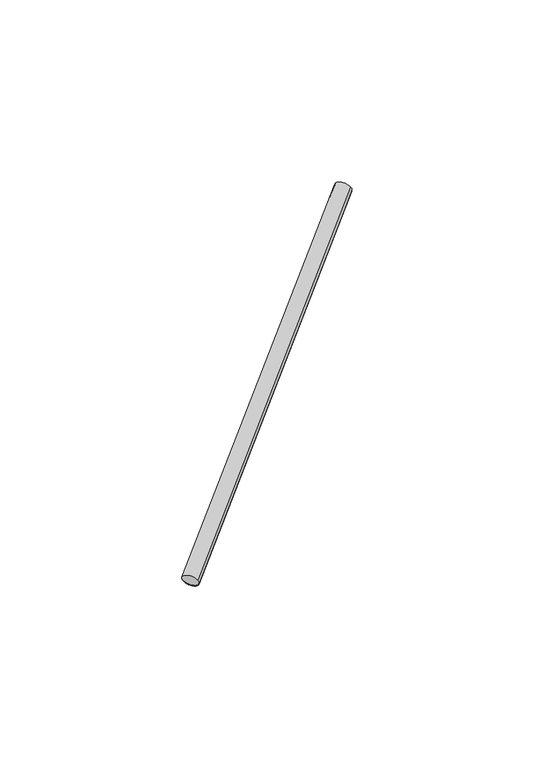
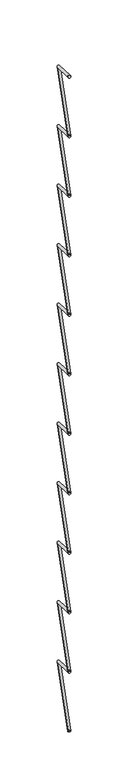
"""IFC4 building model written with IfcOpenShell, lengths in millimetres: proxy geometry, Vigota 2 (Pano 4) (Mf = 837)."""

from ifc_helpers import new_model, si_unit, point, frame, origin, origin_2d, place, context, project, spatial, circle_curve, trimmed, segment, composite_curve, outline, extrude, source, transform, mapped, element, save


def structural_framing_aa4d0655(model_context):
    return source(origin(), model_context, "Body", "SweptSolid", [
        extrude(outline(composite_curve([segment(trimmed(circle_curve(origin_2d(), 2.5), [point((2.5, 0.0))], [point((-2.5, 0.0))], False, "CARTESIAN"), True, "CONTINUOUS"), segment(trimmed(circle_curve(origin_2d(), 2.5), [point((-2.5, 0.0))], [point((2.5, 0.0))], False, "CARTESIAN"), True, "CONTINUOUS")], self_intersect=False)), frame((-42.0, 0.0, 1765.0), z_axis=(0.3218603428886276, 0.8276408817707567, 0.4598004898837537), x_axis=(0.8192319205108605, 3.936835275445103e-11, -0.5734623443750141)), (0.0, 0.0, 1.0), 130.491379),
        extrude(outline(composite_curve([segment(trimmed(circle_curve(origin_2d(), 2.5), [point((2.5, 0.0))], [point((-2.5, 0.0))], False, "CARTESIAN"), True, "CONTINUOUS"), segment(trimmed(circle_curve(origin_2d(), 2.5), [point((-2.5, 0.0))], [point((2.5, 0.0))], False, "CARTESIAN"), True, "CONTINUOUS")], self_intersect=False)), frame((0.0, 108.0, 1825.0), z_axis=(-0.3218603428886276, -0.8276408817707567, 0.4598004898837537), x_axis=(0.8192319205108605, 3.936835275445103e-11, 0.5734623443750141)), (0.0, 0.0, 1.0), 130.491379),
        extrude(outline(composite_curve([segment(trimmed(circle_curve(origin_2d(), 2.5), [point((2.5, 0.0))], [point((-2.5, 0.0))], False, "CARTESIAN"), True, "CONTINUOUS"), segment(trimmed(circle_curve(origin_2d(), 2.5), [point((-2.5, 0.0))], [point((2.5, 0.0))], False, "CARTESIAN"), True, "CONTINUOUS")], self_intersect=False)), frame((-42.0, 0.0, 1885.0), z_axis=(0.3218603428886276, 0.8276408817707567, 0.4598004898837537), x_axis=(0.8192319205108605, 3.936835275445103e-11, -0.5734623443750141)), (0.0, 0.0, 1.0), 130.491379),
        extrude(outline(composite_curve([segment(trimmed(circle_curve(origin_2d(), 2.5), [point((2.5, 0.0))], [point((-2.5, 0.0))], False, "CARTESIAN"), True, "CONTINUOUS"), segment(trimmed(circle_curve(origin_2d(), 2.5), [point((-2.5, 0.0))], [point((2.5, 0.0))], False, "CARTESIAN"), True, "CONTINUOUS")], self_intersect=False)), frame((0.0, 108.0, 1945.0), z_axis=(-0.3218603428886276, -0.8276408817707567, 0.4598004898837537), x_axis=(0.8192319205108605, 3.936835275445103e-11, 0.5734623443750141)), (0.0, 0.0, 1.0), 130.491379),
        extrude(outline(composite_curve([segment(trimmed(circle_curve(origin_2d(), 2.5), [point((2.5, 0.0))], [point((-2.5, 0.0))], False, "CARTESIAN"), True, "CONTINUOUS"), segment(trimmed(circle_curve(origin_2d(), 2.5), [point((-2.5, 0.0))], [point((2.5, 0.0))], False, "CARTESIAN"), True, "CONTINUOUS")], self_intersect=False)), frame((-42.0, 0.0, 2005.0), z_axis=(0.3218603428886276, 0.8276408817707567, 0.4598004898837537), x_axis=(0.8192319205108605, 3.936835275445103e-11, -0.5734623443750141)), (0.0, 0.0, 1.0), 130.491379),
        extrude(outline(composite_curve([segment(trimmed(circle_curve(origin_2d(), 2.5), [point((2.5, 0.0))], [point((-2.5, 0.0))], False, "CARTESIAN"), True, "CONTINUOUS"), segment(trimmed(circle_curve(origin_2d(), 2.5), [point((-2.5, 0.0))], [point((2.5, 0.0))], False, "CARTESIAN"), True, "CONTINUOUS")], self_intersect=False)), frame((0.0, 108.0, 2065.0), z_axis=(-0.3218603428886276, -0.8276408817707567, 0.4598004898837537), x_axis=(0.8192319205108605, 3.936835275445103e-11, 0.5734623443750141)), (0.0, 0.0, 1.0), 130.491379),
        extrude(outline(composite_curve([segment(trimmed(circle_curve(origin_2d(), 2.5), [point((2.5, 0.0))], [point((-2.5, 0.0))], False, "CARTESIAN"), True, "CONTINUOUS"), segment(trimmed(circle_curve(origin_2d(), 2.5), [point((-2.5, 0.0))], [point((2.5, 0.0))], False, "CARTESIAN"), True, "CONTINUOUS")], self_intersect=False)), frame((-42.0, 0.0, 2125.0), z_axis=(0.3218603428886276, 0.8276408817707567, 0.4598004898837537), x_axis=(0.8192319205108605, 3.936835275445103e-11, -0.5734623443750141)), (0.0, 0.0, 1.0), 130.491379),
        extrude(outline(composite_curve([segment(trimmed(circle_curve(origin_2d(), 2.5), [point((2.5, 0.0))], [point((-2.5, 0.0))], False, "CARTESIAN"), True, "CONTINUOUS"), segment(trimmed(circle_curve(origin_2d(), 2.5), [point((-2.5, 0.0))], [point((2.5, 0.0))], False, "CARTESIAN"), True, "CONTINUOUS")], self_intersect=False)), frame((0.0, 108.0, 2185.0), z_axis=(-0.3218603428886276, -0.8276408817707567, 0.4598004898837537), x_axis=(0.8192319205108605, 3.936835275445103e-11, 0.5734623443750141)), (0.0, 0.0, 1.0), 130.491379),
        extrude(outline(composite_curve([segment(trimmed(circle_curve(origin_2d(), 2.5), [point((2.5, 0.0))], [point((-2.5, 0.0))], False, "CARTESIAN"), True, "CONTINUOUS"), segment(trimmed(circle_curve(origin_2d(), 2.5), [point((-2.5, 0.0))], [point((2.5, 0.0))], False, "CARTESIAN"), True, "CONTINUOUS")], self_intersect=False)), frame((-42.0, 0.0, 2245.0), z_axis=(0.3218603428886276, 0.8276408817707567, 0.4598004898837537), x_axis=(0.8192319205108605, 3.936835275445103e-11, -0.5734623443750141)), (0.0, 0.0, 1.0), 130.491379),
        extrude(outline(composite_curve([segment(trimmed(circle_curve(origin_2d(), 2.5), [point((2.5, 0.0))], [point((-2.5, 0.0))], False, "CARTESIAN"), True, "CONTINUOUS"), segment(trimmed(circle_curve(origin_2d(), 2.5), [point((-2.5, 0.0))], [point((2.5, 0.0))], False, "CARTESIAN"), True, "CONTINUOUS")], self_intersect=False)), frame((0.0, 108.0, 2305.0), z_axis=(-0.3218603428886276, -0.8276408817707567, 0.4598004898837537), x_axis=(0.8192319205108605, 3.936835275445103e-11, 0.5734623443750141)), (0.0, 0.0, 1.0), 130.491379),
        extrude(outline(composite_curve([segment(trimmed(circle_curve(origin_2d(), 2.5), [point((2.5, 0.0))], [point((-2.5, 0.0))], False, "CARTESIAN"), True, "CONTINUOUS"), segment(trimmed(circle_curve(origin_2d(), 2.5), [point((-2.5, 0.0))], [point((2.5, 0.0))], False, "CARTESIAN"), True, "CONTINUOUS")], self_intersect=False)), frame((-42.0, 0.0, 2365.0), z_axis=(0.3218603428886276, 0.8276408817707567, 0.4598004898837537), x_axis=(0.8192319205108605, 3.936835275445103e-11, -0.5734623443750141)), (0.0, 0.0, 1.0), 130.491379),
        extrude(outline(composite_curve([segment(trimmed(circle_curve(origin_2d(), 2.5), [point((2.5, 0.0))], [point((-2.5, 0.0))], False, "CARTESIAN"), True, "CONTINUOUS"), segment(trimmed(circle_curve(origin_2d(), 2.5), [point((-2.5, 0.0))], [point((2.5, 0.0))], False, "CARTESIAN"), True, "CONTINUOUS")], self_intersect=False)), frame((0.0, 108.0, 2425.0), z_axis=(-0.3218603428886276, -0.8276408817707567, 0.4598004898837537), x_axis=(0.8192319205108605, 3.936835275445103e-11, 0.5734623443750141)), (0.0, 0.0, 1.0), 130.491379),
        extrude(outline(composite_curve([segment(trimmed(circle_curve(origin_2d(), 2.5), [point((2.5, 0.0))], [point((-2.5, 0.0))], False, "CARTESIAN"), True, "CONTINUOUS"), segment(trimmed(circle_curve(origin_2d(), 2.5), [point((-2.5, 0.0))], [point((2.5, 0.0))], False, "CARTESIAN"), True, "CONTINUOUS")], self_intersect=False)), frame((-42.0, 0.0, 2485.0), z_axis=(0.3218603428886276, 0.8276408817707567, 0.4598004898837537), x_axis=(0.8192319205108605, 3.936835275445103e-11, -0.5734623443750141)), (0.0, 0.0, 1.0), 130.491379),
        extrude(outline(composite_curve([segment(trimmed(circle_curve(origin_2d(), 2.5), [point((2.5, 0.0))], [point((-2.5, 0.0))], False, "CARTESIAN"), True, "CONTINUOUS"), segment(trimmed(circle_curve(origin_2d(), 2.5), [point((-2.5, 0.0))], [point((2.5, 0.0))], False, "CARTESIAN"), True, "CONTINUOUS")], self_intersect=False)), frame((0.0, 108.0, 2545.0), z_axis=(-0.3218603428886276, -0.8276408817707567, 0.4598004898837537), x_axis=(0.8192319205108605, 3.936835275445103e-11, 0.5734623443750141)), (0.0, 0.0, 1.0), 130.491379),
        extrude(outline(composite_curve([segment(trimmed(circle_curve(origin_2d(), 2.5), [point((2.5, 0.0))], [point((-2.5, 0.0))], False, "CARTESIAN"), True, "CONTINUOUS"), segment(trimmed(circle_curve(origin_2d(), 2.5), [point((-2.5, 0.0))], [point((2.5, 0.0))], False, "CARTESIAN"), True, "CONTINUOUS")], self_intersect=False)), frame((-42.0, 0.0, 2605.0), z_axis=(0.3218603428886276, 0.8276408817707567, 0.4598004898837537), x_axis=(0.8192319205108605, 3.936835275445103e-11, -0.5734623443750141)), (0.0, 0.0, 1.0), 130.491379),
        extrude(outline(composite_curve([segment(trimmed(circle_curve(origin_2d(), 2.5), [point((2.5, 0.0))], [point((-2.5, 0.0))], False, "CARTESIAN"), True, "CONTINUOUS"), segment(trimmed(circle_curve(origin_2d(), 2.5), [point((-2.5, 0.0))], [point((2.5, 0.0))], False, "CARTESIAN"), True, "CONTINUOUS")], self_intersect=False)), frame((0.0, 108.0, 2665.0), z_axis=(-0.3218603428886276, -0.8276408817707567, 0.4598004898837537), x_axis=(0.8192319205108605, 3.936835275445103e-11, 0.5734623443750141)), (0.0, 0.0, 1.0), 130.491379),
        extrude(outline(composite_curve([segment(trimmed(circle_curve(origin_2d(), 2.5), [point((2.5, 0.0))], [point((-2.5, 0.0))], False, "CARTESIAN"), True, "CONTINUOUS"), segment(trimmed(circle_curve(origin_2d(), 2.5), [point((-2.5, 0.0))], [point((2.5, 0.0))], False, "CARTESIAN"), True, "CONTINUOUS")], self_intersect=False)), frame((-42.0, 0.0, 2725.0), z_axis=(0.3218603428886276, 0.8276408817707567, 0.4598004898837537), x_axis=(0.8192319205108605, 3.936835275445103e-11, -0.5734623443750141)), (0.0, 0.0, 1.0), 130.491379),
        extrude(outline(composite_curve([segment(trimmed(circle_curve(origin_2d(), 2.5), [point((2.5, 0.0))], [point((-2.5, 0.0))], False, "CARTESIAN"), True, "CONTINUOUS"), segment(trimmed(circle_curve(origin_2d(), 2.5), [point((-2.5, 0.0))], [point((2.5, 0.0))], False, "CARTESIAN"), True, "CONTINUOUS")], self_intersect=False)), frame((0.0, 108.0, 2785.0), z_axis=(-0.3218603428886276, -0.8276408817707567, 0.4598004898837537), x_axis=(0.8192319205108605, 3.936835275445103e-11, 0.5734623443750141)), (0.0, 0.0, 1.0), 130.491379),
        extrude(outline(composite_curve([segment(trimmed(circle_curve(origin_2d(), 2.5), [point((2.5, 0.0))], [point((-2.5, 0.0))], False, "CARTESIAN"), True, "CONTINUOUS"), segment(trimmed(circle_curve(origin_2d(), 2.5), [point((-2.5, 0.0))], [point((2.5, 0.0))], False, "CARTESIAN"), True, "CONTINUOUS")], self_intersect=False)), frame((-42.0, 0.0, 2845.0), z_axis=(0.3218603428886276, 0.8276408817707567, 0.4598004898837537), x_axis=(0.8192319205108605, 3.936835275445103e-11, -0.5734623443750141)), (0.0, 0.0, 1.0), 130.491379),
        extrude(outline(composite_curve([segment(trimmed(circle_curve(origin_2d(), 2.5), [point((2.5, 0.0))], [point((-2.5, 0.0))], False, "CARTESIAN"), True, "CONTINUOUS"), segment(trimmed(circle_curve(origin_2d(), 2.5), [point((-2.5, 0.0))], [point((2.5, 0.0))], False, "CARTESIAN"), True, "CONTINUOUS")], self_intersect=False)), frame((0.0, 108.0, 2905.0), z_axis=(-0.3218603428886276, -0.8276408817707567, 0.4598004898837537), x_axis=(0.8192319205108605, 3.936835275445103e-11, 0.5734623443750141)), (0.0, 0.0, 1.0), 130.491379),
        extrude(outline(composite_curve([segment(trimmed(circle_curve(origin_2d(), 2.5), [point((2.5, 0.0))], [point((-2.5, 0.0))], False, "CARTESIAN"), True, "CONTINUOUS"), segment(trimmed(circle_curve(origin_2d(), 2.5), [point((-2.5, 0.0))], [point((2.5, 0.0))], False, "CARTESIAN"), True, "CONTINUOUS")], self_intersect=False)), frame((-42.0, 0.0, 2965.0), z_axis=(0.3218603428886276, 0.8276408817707567, 0.4598004898837537), x_axis=(0.8192319205108605, 3.936835275445103e-11, -0.5734623443750141)), (0.0, 0.0, 1.0), 130.491379),
        extrude(outline(composite_curve([segment(trimmed(circle_curve(origin_2d(), 2.5), [point((2.5, 0.0))], [point((-2.5, 0.0))], False, "CARTESIAN"), True, "CONTINUOUS"), segment(trimmed(circle_curve(origin_2d(), 2.5), [point((-2.5, 0.0))], [point((2.5, 0.0))], False, "CARTESIAN"), True, "CONTINUOUS")], self_intersect=False)), frame((0.0, 108.0, 3025.0), z_axis=(-0.3218603428886276, -0.8276408817707567, 0.4598004898837537), x_axis=(0.8192319205108605, 3.936835275445103e-11, 0.5734623443750141)), (0.0, 0.0, 1.0), 130.491379),
    ])


if __name__ == "__main__":
    model = new_model("IFC4")
    model_context = context("Model", 3, world=origin())
    ifc_project = project(units=[si_unit("LENGTHUNIT", "METRE", prefix="MILLI")], contexts=[model_context])
    site = spatial("IfcSite", under=ifc_project)
    building = spatial("IfcBuilding", under=site)
    placement = place(None, origin())
    structural_framing_shape = structural_framing_aa4d0655(model_context)
    element("IfcBuildingElementProxy", 1, Name="Vigota 2 (Pano 4) (Mf = 837)", ObjectType="Vigota 2 (Pano 4) (Mf = 837)", at=placement, inside=building, context=model_context, shape_type="MappedRepresentation", body=[
        mapped(structural_framing_shape, transform((0.0, 0.0, 0.0), x_axis=(1.0, 0.0, 0.0), y_axis=(0.0, 1.0, 0.0), z_axis=(0.0, 0.0, 1.0))),
    ])
    save(model, "model.ifc")

# Revit data of these elements
# Element 1 (IfcBuildingElementProxy, "Vigota 2 (Pano 4) (Mf = 837)")
#   Materials on its faces: "Aço", "Concreto armado"
# Materials
#   "Aço": class "Metal", colour RGB 120 120 120, transparency 0, Description = "Aço estrutural A36 grau, ASTM B, acabamento laminado", Cost = 0
#   "Concreto armado": class "Não atribuído", colour RGB 168 169 158, transparency 0
